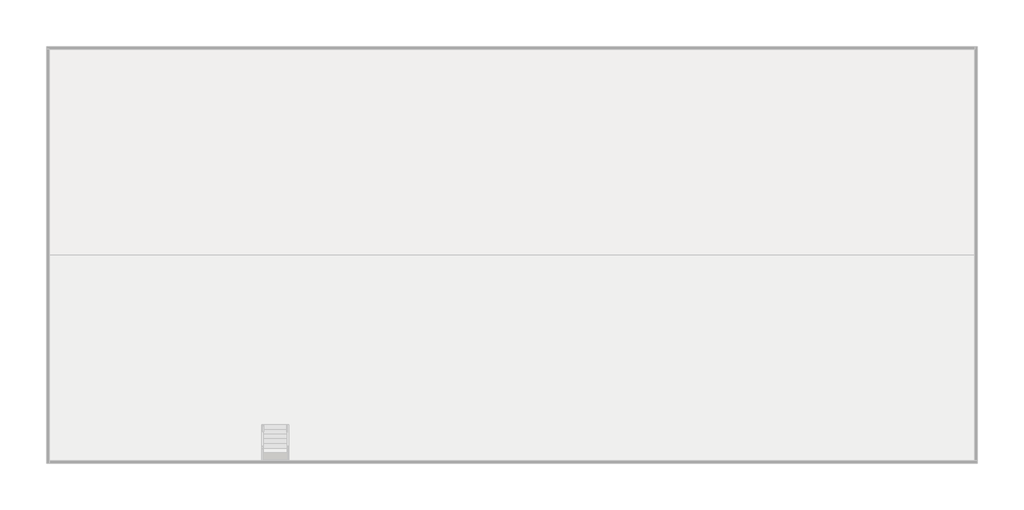
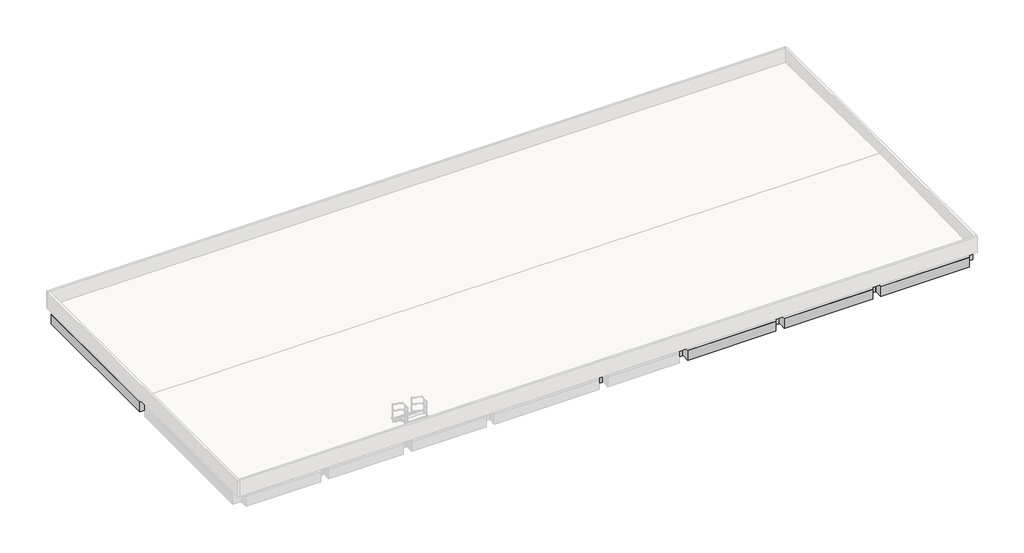
# One storey, part 2 of 3: 33 beams.
# Revit data of these elements (continued)
# Type "RC Beam_Rectangular : H_SB_AR_S16_B400xH900_RB1" (continued)
#   H_WM Code_4 = "A04AM078-00002 |  | M2 | Finishing Work | Painting Work | Internal Wall Painting | Water Emulsion Paint |  |  |  | A04AM078-00002 Finishing Work Painting Work Internal Wall Painting Water Emulsion Paint        |"
#   중앙부 하부근 = ""
#   중앙부 상부근 = ""
#   중앙부 보조근 = ""
#   중앙부 늑근 = ""
#   외단부 하부근 = ""
#   외단부 상부근 = ""
#   외단부 보조근 = ""
#   외단부 늑근 = ""
#   부호 = "TG3"
#   내단부 하부근 = ""
#   내단부 상부근 = ""
#   내단부 보조근 = ""
#   내단부 늑근 = ""
#   ALL 하부근 = "3-D20"
#   ALL 상부근 = "3-D20"
#   ALL 보조근 = ""
#   ALL 늑근 = "2-D10 @120"
#   Width = 400 mm
#   Height = 900 mm
#   Length [instance default] = 1524 mm
#   b = 400 mm
#   h = 900 mm
#   hec_material3 [instance default] = none
#   hec_material2 [instance default] = none
#   hec_material1 [instance default] = none
#   Structural Material [instance default] = none
#   Assembly Code = ""
# Type "RC Beam_Rectangular : H_SB_AR_S16_B600xH900_RB2"
#   H_Q'ty Cal Type Tag = "SB-Q1"
#   H_WM Code_1 = "A03AF032-00010 |  | M3 | Concrete Work | Superstructure Work | Structural Concrete | Cement Type-1 | 20MPa < F'c (Cylinder Strength) ≤ 25MPa |  |  |  | A03AF032-00010 Concrete Work Superstructure Work Structural Concrete  Cement Type-1 20MPa < F'c (Cylinder Strength) ≤ 25MPa      |  F'c (Cylinder Strength) = 24MPa"
#   H_WM Code_2 = "A03AD037-00002 |  | TON | Concrete Work | Substructure Work | Rebar Work | Deformed Bar (Non-Coat.) | 400MPa<Fy≤470MPa |  |  |  | A03AD037-00002 Concrete Work Substructure Work Rebar Work Deformed Bar (Non-Coat.)  400MPa<Fy≤470MPa      | ASTM A615 GRADE 60 (Fy=420MPa)"
#   H_WM Code_3 = "A03AF036-00001 |  | M2 | Concrete Work | Superstructure Work | Form Work (1 time in use) | Flat Form | Dressed Lumber, Plywood or Steel Form(Wood Planks are not Allowed) incl. Chamfer |  |  | A03AF036-00001 Concrete Work Superstructure Work Form Work (1 time in use) Flat Form     Dressed Lumber, Plywood or Steel Form(Wood Planks are not Allowed) incl. Chamfer   |"
#   H_WM Code_4 = "A04AM078-00002 |  | M2 | Finishing Work | Painting Work | Internal Wall Painting | Water Emulsion Paint |  |  |  | A04AM078-00002 Finishing Work Painting Work Internal Wall Painting Water Emulsion Paint        |"
#   중앙부 하부근 = ""
#   중앙부 상부근 = ""
#   중앙부 보조근 = ""
#   중앙부 늑근 = ""
#   외단부 하부근 = ""
#   외단부 상부근 = ""
#   외단부 보조근 = ""
#   외단부 늑근 = ""
#   부호 = "TG3"
#   내단부 하부근 = ""
#   내단부 상부근 = ""
#   내단부 보조근 = ""
#   내단부 늑근 = ""
#   ALL 하부근 = "3-D20"
#   ALL 상부근 = "3-D20"
#   ALL 보조근 = ""
#   ALL 늑근 = "2-D10 @120"
#   Width = 600 mm
#   Height = 900 mm
#   Length [instance default] = 1524 mm
#   b = 600 mm
#   h = 900 mm
#   hec_material3 [instance default] = none
#   hec_material2 [instance default] = none
#   hec_material1 [instance default] = none
#   Structural Material [instance default] = none
#   Assembly Code = ""
# Type "RC Beam_Rectangular : H_SB_AR_S16_B600xH900_RB3"
#   H_Q'ty Cal Type Tag = "CE-Q1"
#   중앙부 하부근 = ""
#   중앙부 상부근 = ""
#   중앙부 보조근 = ""
#   중앙부 늑근 = ""
#   외단부 하부근 = ""
#   외단부 상부근 = ""
#   외단부 보조근 = ""
#   외단부 늑근 = ""
#   부호 = "TG3"
#   내단부 하부근 = ""
#   내단부 상부근 = ""
#   내단부 보조근 = ""
#   내단부 늑근 = ""
#   ALL 하부근 = "3-D20"
#   ALL 상부근 = "3-D20"
#   ALL 보조근 = ""
#   ALL 늑근 = "2-D10 @120"
#   Width = 600 mm
#   Height = 900 mm
#   Length [instance default] = 1524 mm
#   b = 600 mm
#   h = 900 mm
#   hec_material3 [instance default] = none
#   hec_material2 [instance default] = none
#   hec_material1 [instance default] = none
#   Structural Material [instance default] = none
#   Assembly Code = ""
# Elements 1, 2, 3, 4, 5, 10, 11, 12 (IfcBeam, "RC Beam_Rectangular : H_SB_AR_S16_B600xH900_RG9")
#   Comments = ""
#   hec_material3 = none
#   hec_material2 = none
#   hec_material1 = none
#   Structural Material = Concrete - Cast-in-Place Concrete - 35 MPa
#   Phase Created = New Construction
#   Materials on its faces: "Concrete - Cast-in-Place Concrete - 35 MPa"
# Elements 6, 7, 8, 9 (IfcBeam, "RC Beam_Rectangular : H_SB_AR_S16_B600xH900_RG5")
#   Comments = ""
#   hec_material3 = none
#   hec_material2 = none
#   hec_material1 = none
#   Structural Material = Concrete - Cast-in-Place Concrete - 35 MPa
#   Phase Created = New Construction
#   Materials on its faces: "Concrete - Cast-in-Place Concrete - 35 MPa"
# Element 13 (IfcBeam, "RC Beam_Rectangular : H_SB_AR_S16_B600xH900_RG6")
#   Comments = ""
#   hec_material3 = none
#   hec_material2 = none
#   hec_material1 = none
#   Structural Material = Concrete - Cast-in-Place Concrete - 35 MPa
#   Phase Created = New Construction
#   Materials on its faces: "Concrete - Cast-in-Place Concrete - 35 MPa"
# Elements 14, 15 (IfcBeam, "RC Beam_Rectangular : H_SB_AR_S16_B400xH900_RG1")
#   Comments = ""
#   hec_material3 = none
#   hec_material2 = none
#   hec_material1 = none
#   Structural Material = Concrete - Cast-in-Place Concrete - 35 MPa
#   Phase Created = New Construction
#   Materials on its faces: "Concrete - Cast-in-Place Concrete - 35 MPa"
# Element 16 (IfcBeam, "RC Beam_Rectangular : H_SB_AR_S16_B600xH900_RG1A")
#   Comments = ""
#   hec_material3 = none
#   hec_material2 = none
#   hec_material1 = none
#   Structural Material = Concrete - Cast-in-Place Concrete - 35 MPa
#   Phase Created = New Construction
#   Materials on its faces: "Concrete - Cast-in-Place Concrete - 35 MPa"
# Elements 17, 19, 21, 22 (IfcBeam, "RC Beam_Rectangular : H_SB_AR_S16_B500xH900_RG3")
#   Comments = ""
#   hec_material3 = none
#   hec_material2 = none
#   hec_material1 = none
#   Structural Material = Concrete - Cast-in-Place Concrete - 35 MPa
#   Phase Created = New Construction
#   Materials on its faces: "Concrete - Cast-in-Place Concrete - 35 MPa"
# Elements 18, 20 (IfcBeam, "RC Beam_Rectangular : H_SB_AR_S16_B500xH900_RG2")
#   Comments = ""
#   hec_material3 = none
#   hec_material2 = none
#   hec_material1 = none
#   Structural Material = Concrete - Cast-in-Place Concrete - 35 MPa
#   Phase Created = New Construction
#   Materials on its faces: "Concrete - Cast-in-Place Concrete - 35 MPa"
# Element 23 (IfcBeam, "RC Beam_Rectangular : H_SB_AR_S16_B600xH900_RG8")
#   Comments = ""
#   hec_material3 = none
#   hec_material2 = none
#   hec_material1 = none
#   Structural Material = Concrete - Cast-in-Place Concrete - 35 MPa
#   Phase Created = New Construction
#   Materials on its faces: "Concrete - Cast-in-Place Concrete - 35 MPa"
# Element 24 (IfcBeam, "RC Beam_Rectangular : H_SB_AR_S16_B600xH900_RG5A")
#   hec_material3 = none
#   hec_material2 = none
#   hec_material1 = none
#   Structural Material = Concrete - Cast-in-Place Concrete - 35 MPa
#   Phase Created = New Construction
#   Materials on its faces: "Concrete - Cast-in-Place Concrete - 35 MPa"
# Elements 25, 26, 27 (IfcBeam, "RC Beam_Rectangular : H_SB_AR_S16_B400xH900_RB1")
#   hec_material3 = none
#   hec_material2 = none
#   hec_material1 = none
#   Structural Material = Concrete - Cast-in-Place Concrete - 35 MPa
#   Phase Created = New Construction
#   Materials on its faces: "Concrete - Cast-in-Place Concrete - 35 MPa"
# Elements 28, 29 (IfcBeam, "RC Beam_Rectangular : H_SB_AR_S16_B600xH900_RB2")
#   hec_material3 = none
#   hec_material2 = none
#   hec_material1 = none
#   Structural Material = Concrete - Cast-in-Place Concrete - 35 MPa
#   Phase Created = New Construction
#   Materials on its faces: "Concrete - Cast-in-Place Concrete - 35 MPa"
# Elements 30, 31, 32, 33 (IfcBeam, "RC Beam_Rectangular : H_SB_AR_S16_B600xH900_RB3")
#   hec_material3 = none
#   hec_material2 = none
#   hec_material1 = none
#   Structural Material = Concrete - Cast-in-Place Concrete - 35 MPa
#   Phase Created = New Construction
#   Materials on its faces: "Concrete - Cast-in-Place Concrete - 35 MPa"
# Materials
#   "Concrete - Cast-in-Place Concrete - 35 MPa": class "Concrete", colour RGB 192 192 192, transparency 0, Description = "ACRYLIC EMULSION PAINT ON THK.13 CEMENT PLASTER", Cost = 0
